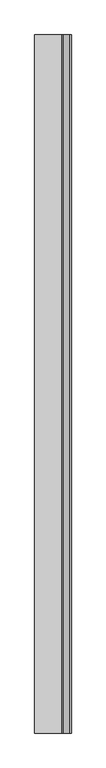
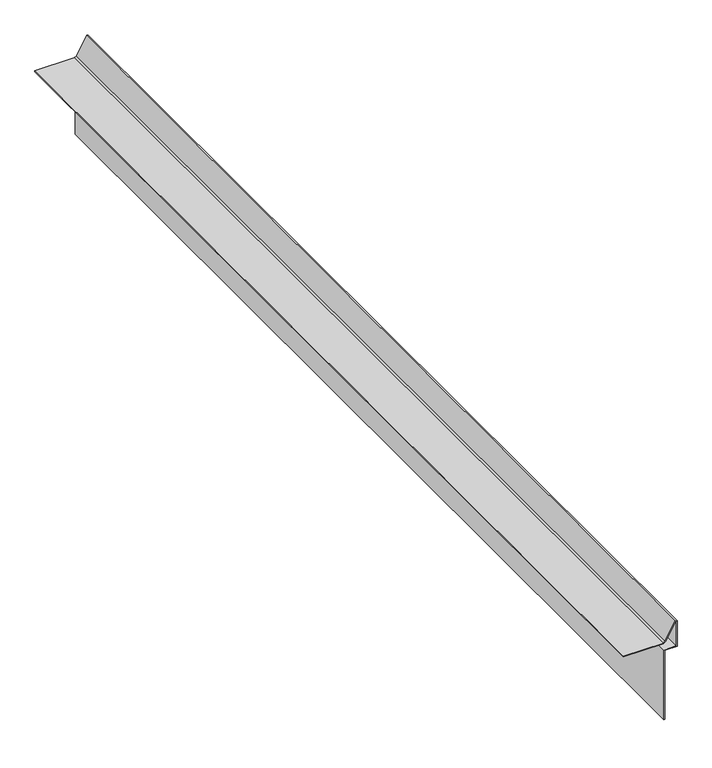
"""IFC4 building model written with IfcOpenShell, lengths in millimetres: proxy geometry, GRAVEL STOP13:GRAVEL STOP002:305288 : GRAVEL STOP13:GRAVEL STOP002:305288."""

from ifc_helpers import new_model, si_unit, frame, origin, place, context, project, spatial, polyline, outline, extrude, source, transform, mapped, element, save


def generic_models_c66da025(model_context):
    return source(origin(), model_context, "Body", "SweptSolid", [
        extrude(outline(polyline([(40294.5307525, 415.3370458), (40295.3431515, 412.3051314), (40259.5408757, 391.6346779), (40257.3744784, 387.8823677), (40257.3744784, 310.424461), (40255.9633674, 310.424461), (40255.9633674, 388.2604737), (40258.5078708, 392.6676828), (40293.699878, 412.9857976), (40293.447969, 413.9259348), (40242.3744784, 413.9259348), (40242.3744784, 389.5861972), (40097.9858473, 389.5861972), (40097.9858473, 390.9973082), (40240.9633674, 390.9973082), (40240.9633674, 415.3370458), (40294.5307525, 415.3370458)])), frame((0.0, -774.5581162, 0.0), z_axis=(0.0, 1.0, 0.0), x_axis=(0.0, 0.0, 1.0)), (0.0, 0.0, 1.0), 2000.25),
    ])


if __name__ == "__main__":
    model = new_model("IFC4")
    model_context = context("Model", 3, world=origin())
    ifc_project = project(units=[si_unit("LENGTHUNIT", "METRE", prefix="MILLI")], contexts=[model_context])
    site = spatial("IfcSite", under=ifc_project)
    building = spatial("IfcBuilding", under=site)
    placement = place(None, origin())
    generic_models_shape = generic_models_c66da025(model_context)
    element("IfcBuildingElementProxy", 1, Name="GRAVEL STOP13:GRAVEL STOP002:305288 : GRAVEL STOP13:GRAVEL STOP002:305288", ObjectType="GRAVEL STOP13:GRAVEL STOP002:305288 : GRAVEL STOP13:GRAVEL STOP002:305288", at=placement, inside=building, context=model_context, shape_type="MappedRepresentation", body=[
        mapped(generic_models_shape, transform((0.0, 0.0, 0.0), x_axis=(1.0, 0.0, 0.0), y_axis=(0.0, 1.0, 0.0), z_axis=(0.0, 0.0, 1.0))),
    ])
    save(model, "model.ifc")

# Revit data of these elements
# Type "GRAVEL STOP13:GRAVEL STOP002:305288 : GRAVEL STOP13:GRAVEL STOP002:305288"
#   NameOverride = "GRAVEL STOP13:GRAVEL STOP002:305288"
#   ObjectTypeOverride = "GRAVEL STOP13:GRAVEL STOP002"
#   Reference = "GRAVEL STOP002"
#   Category = "Generic Models"
#   Tag = "305288"
# Element 1 (IfcBuildingElementProxy, "GRAVEL STOP13:GRAVEL STOP002:305288 : GRAVEL STOP13:GRAVEL STOP002:305288")
#   Materials on its faces: "GRAVEL STOP REQUIRED WITH GRAVEL SURFACE SYSTEMS"
# Materials
#   "GRAVEL STOP REQUIRED WITH GRAVEL SURFACE SYSTEMS": class "Unassigned", colour RGB 170 170 127, transparency 0, Cost = 0
